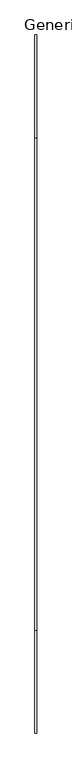
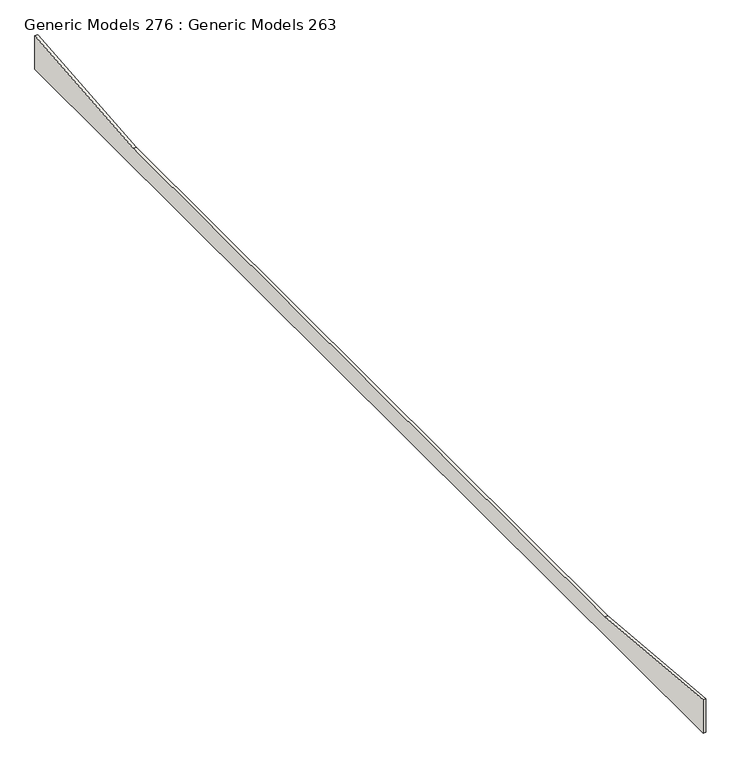
"""IFC4 building model written with IfcOpenShell, lengths in millimetres: wall geometry, Generic Models 276 : Generic Models 263."""

from ifc_helpers import new_model, si_unit, frame, origin, place, context, project, spatial, polyline, outline, extrude, source, transform, mapped, element, save


def generic_models_276_generic_models_263_4ecf39a9(model_context):
    return source(origin(), model_context, "Body", "SweptSolid", [
        extrude(outline(polyline([(2106.5727422, 2.0699085), (2106.5727422, -314.8198762), (-8256.6272578, -314.8198762), (-8256.6272578, 2.0699085), (-6732.6272578, -137.0198762), (582.5727422, -137.0198762), (2106.5727422, 2.0699085)])), frame((91554.5797726, 0.0, 0.0), z_axis=(1.0, 0.0, 0.0), x_axis=(0.0, 1.0, 0.0)), (0.0, 0.0, 1.0), 25.4),
    ])


if __name__ == "__main__":
    model = new_model("IFC4")
    model_context = context("Model", 3, world=origin())
    ifc_project = project(units=[si_unit("LENGTHUNIT", "METRE", prefix="MILLI")], contexts=[model_context])
    site = spatial("IfcSite", under=ifc_project)
    building = spatial("IfcBuilding", under=site)
    placement = place(None, origin())
    generic_models_276_generic_models_263_shape = generic_models_276_generic_models_263_4ecf39a9(model_context)
    element("IfcWall", 1, ObjectType="Generic Models 276 : Generic Models 263", at=placement, inside=building, context=model_context, shape_type="MappedRepresentation", body=[
        mapped(generic_models_276_generic_models_263_shape, transform((0.0, 0.0, 0.0), x_axis=(1.0, 0.0, 0.0), y_axis=(0.0, 1.0, 0.0), z_axis=(0.0, 0.0, 1.0))),
    ])
    save(model, "model.ifc")

# Revit data of these elements
# Element 1 (IfcWall, "Generic Models 276 : Generic Models 263")
#   Materials on its faces: "1\" EXPANSION JOINT"
# Materials
#   "1\" EXPANSION JOINT": class "Concrete", colour RGB 197 197 197, transparency 0, Description = "Cast-in-place concrete", Cost = 0
